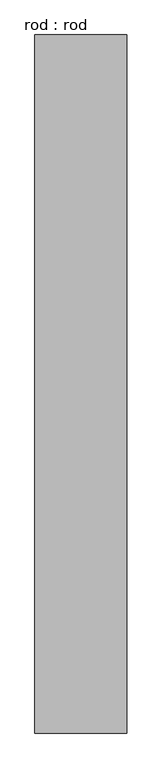
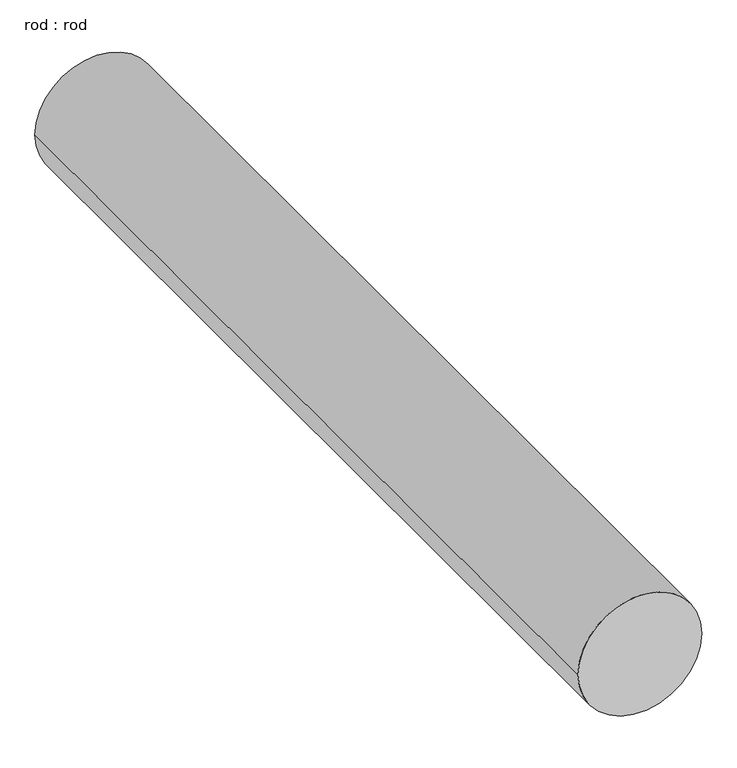
"""IFC4 building model written with IfcOpenShell, lengths in millimetres: proxy geometry, rod : rod."""

from ifc_helpers import new_model, si_unit, point, frame, frame_2d, origin, place, context, project, spatial, circle_curve, trimmed, segment, composite_curve, outline, extrude, source, transform, mapped, element, save


def rod_rod_df166a33(model_context):
    return source(origin(), model_context, "Body", "SweptSolid", [
        extrude(outline(composite_curve([segment(trimmed(circle_curve(frame_2d((0.0108462, 0.0)), 200.0), [point((0.0108462, 200.0))], [point((0.0108462, -200.0))], False, "CARTESIAN"), True, "CONTINUOUS"), segment(trimmed(circle_curve(frame_2d((0.0108462, 0.0)), 200.0), [point((0.0108462, -200.0))], [point((0.0108462, 200.0))], False, "CARTESIAN"), True, "CONTINUOUS")], self_intersect=False)), frame((0.0, 2572.7286153, 0.0), z_axis=(0.0, 1.0, 0.0), x_axis=(0.0, 0.0, 1.0)), (0.0, 0.0, 1.0), 3040.0),
    ])


if __name__ == "__main__":
    model = new_model("IFC4")
    model_context = context("Model", 3, world=origin())
    ifc_project = project(units=[si_unit("LENGTHUNIT", "METRE", prefix="MILLI")], contexts=[model_context])
    site = spatial("IfcSite", under=ifc_project)
    building = spatial("IfcBuilding", under=site)
    placement = place(None, origin())
    rod_rod_shape = rod_rod_df166a33(model_context)
    element("IfcBuildingElementProxy", 1, Name="rod : rod", ObjectType="rod : rod", at=placement, inside=building, context=model_context, shape_type="MappedRepresentation", body=[
        mapped(rod_rod_shape, transform((0.0, 0.0, 0.0), x_axis=(1.0, 0.0, 0.0), y_axis=(0.0, 1.0, 0.0), z_axis=(0.0, 0.0, 1.0))),
    ])
    save(model, "model.ifc")

# Revit data of these elements
# Type "rod : rod"
#   Default Elevation = 0
